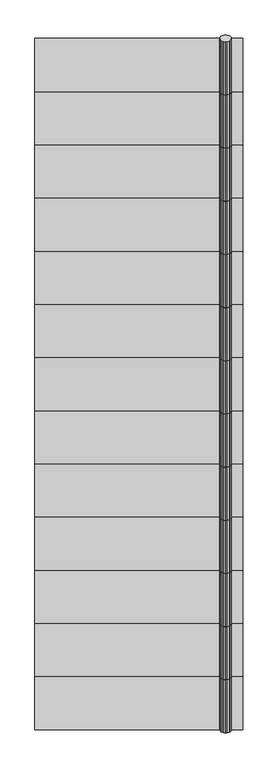
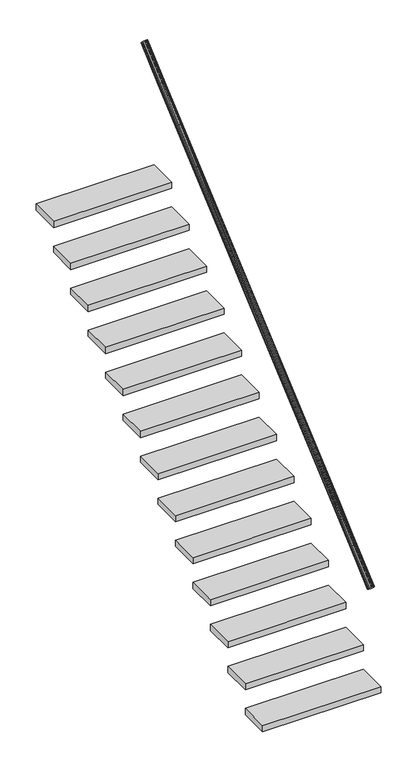
"""IFC4 building model written with IfcOpenShell, lengths in millimetres: stair geometry, 0_3d_modell."""

import ifcopenshell
import ifcopenshell.guid

model = None  # the IFC model being written
_history = None  # IfcOwnerHistory: only IFC2X3 demands one
_inside = {}  # id of a spatial element -> (the spatial element, [elements in it])
_under = {}  # id of a project, library or spatial element -> (it, [spatial elements below it])
_declared = {}  # id of a project -> (the project, [libraries it declares])
_typed = {}  # id of a type object -> (the type object, [elements of that type])
_made_of = {}  # id of a material, layer set ... -> (it, [elements and type objects made of it])


def new_model(schema):
    """Start an empty IFC model of exactly this schema.

    Asked for "IFC4X3", IfcOpenShell would pick the latest addendum, in which some entities
    have other attributes; the version numbers below select the first issue.
    IFC2X3 requires an IfcOwnerHistory on every rooted entity: one is made here for all.
    """
    global model, _history
    if schema == "IFC4X3":
        model = ifcopenshell.file(schema_version=(4, 3, 0, 0))
    else:
        model = ifcopenshell.file(schema=schema)
    _inside.clear()
    _under.clear()
    _declared.clear()
    _typed.clear()
    _made_of.clear()
    _history = None
    if model.schema == "IFC2X3":
        org = make("IfcOrganization", Name="unknown")
        user = make(
            "IfcPersonAndOrganization",
            ThePerson=make("IfcPerson", FamilyName="unknown"),
            TheOrganization=org,
        )
        app = make(
            "IfcApplication",
            ApplicationDeveloper=org,
            Version="unknown",
            ApplicationFullName="unknown",
            ApplicationIdentifier="unknown",
        )
        _history = make(
            "IfcOwnerHistory",
            OwningUser=user,
            OwningApplication=app,
            ChangeAction="ADDED",
            CreationDate=0,
        )
    return model


def make(cls, **values):
    """One entity of the class cls with the attributes given. An attribute that is None is left unset."""
    return model.create_entity(
        cls, **{name: value for name, value in values.items() if value is not None}
    )


def rooted(cls, **values):
    """An entity with a GlobalId (a new one), such as an element, a storey or a relation."""
    return make(cls, GlobalId=ifcopenshell.guid.new(), OwnerHistory=_history, **values)


def si_unit(unit_type, name, prefix=None):
    """IfcSIUnit, for example si_unit("LENGTHUNIT", "METRE", prefix="MILLI")."""
    return make("IfcSIUnit", UnitType=unit_type, Prefix=prefix, Name=name)


def assignment(units):
    """IfcUnitAssignment: the units of a project."""
    return None if units is None else make("IfcUnitAssignment", Units=units)


def point(xyz):
    """IfcCartesianPoint."""
    return None if xyz is None else make("IfcCartesianPoint", Coordinates=xyz)


def direction(xyz):
    """IfcDirection."""
    return None if xyz is None else make("IfcDirection", DirectionRatios=xyz)


def frame(location, z_axis=None, x_axis=None):
    """IfcAxis2Placement3D, a coordinate frame: its origin and axes. An axis left out is left unset."""
    return make(
        "IfcAxis2Placement3D",
        Location=point(location),
        Axis=direction(z_axis),
        RefDirection=direction(x_axis),
    )


def origin():
    """The frame at (0, 0, 0) with its axes left unset."""
    return frame((0.0, 0.0, 0.0))


def origin_with_axes():
    """The frame at (0, 0, 0) with the z axis (0, 0, 1) and the x axis (1, 0, 0) written out."""
    return frame((0.0, 0.0, 0.0), z_axis=(0.0, 0.0, 1.0), x_axis=(1.0, 0.0, 0.0))


def place(relative_to, where):
    """IfcLocalPlacement: puts the frame where relative to a parent placement (None: the world)."""
    return make(
        "IfcLocalPlacement", PlacementRelTo=relative_to, RelativePlacement=where
    )


def context(
    kind, dimensions, precision=None, world=None, true_north=None, identifier=None
):
    """IfcGeometricRepresentationContext, for example the 3D "Model" context."""
    return make(
        "IfcGeometricRepresentationContext",
        ContextIdentifier=identifier,
        ContextType=kind,
        CoordinateSpaceDimension=dimensions,
        Precision=precision,
        WorldCoordinateSystem=world,
        TrueNorth=true_north,
    )


def project(units=None, contexts=None):
    """IfcProject with its units and contexts."""
    return rooted(
        "IfcProject",
        Name="project",
        RepresentationContexts=contexts,
        UnitsInContext=assignment(units),
    )


def spatial(cls, under=None, at=None, **own):
    """A site, building, storey or space (cls), placed at a placement, below another one or the project."""
    s = rooted(cls, ObjectPlacement=at, **own)
    if under is not None:
        _under.setdefault(under.id(), (under, []))[1].append(s)
    return s


def polyline(points):
    """IfcPolyline through the points."""
    return make("IfcPolyline", Points=[point(p) for p in points])


def outline(outer, holes=None, kind="AREA"):
    """IfcArbitraryClosedProfileDef: a profile drawn as a closed curve; with holes, ...WithVoids."""
    if holes is None:
        return make("IfcArbitraryClosedProfileDef", ProfileType=kind, OuterCurve=outer)
    return make(
        "IfcArbitraryProfileDefWithVoids",
        ProfileType=kind,
        OuterCurve=outer,
        InnerCurves=holes,
    )


def extrude(swept, where, along, depth):
    """IfcExtrudedAreaSolid: the profile swept, set in the frame where, extruded along a direction by depth."""
    return make(
        "IfcExtrudedAreaSolid",
        SweptArea=swept,
        Position=where,
        ExtrudedDirection=direction(along),
        Depth=depth,
    )


def shape(context_of_items, identifier, shape_type, items):
    """IfcShapeRepresentation: the items that make up one representation, for example the "Body"."""
    return make(
        "IfcShapeRepresentation",
        ContextOfItems=context_of_items,
        RepresentationIdentifier=identifier,
        RepresentationType=shape_type,
        Items=items,
    )


def source(mapping_origin, context_of_items, identifier, shape_type, items):
    """IfcRepresentationMap: a shape defined once, which mapped items show again and again."""
    return make(
        "IfcRepresentationMap",
        MappingOrigin=mapping_origin,
        MappedRepresentation=shape(context_of_items, identifier, shape_type, items),
    )


def transform(
    local_origin,
    x_axis=None,
    y_axis=None,
    z_axis=None,
    scale=None,
    scale2=None,
    scale3=None,
    uniform=True,
):
    """IfcCartesianTransformationOperator3D, or its non-uniform kind. x_axis, y_axis, z_axis: its Axis1, 2, 3."""
    if uniform:
        return make(
            "IfcCartesianTransformationOperator3D",
            Axis1=direction(x_axis),
            Axis2=direction(y_axis),
            LocalOrigin=point(local_origin),
            Scale=scale,
            Axis3=direction(z_axis),
        )
    return make(
        "IfcCartesianTransformationOperator3DnonUniform",
        Axis1=direction(x_axis),
        Axis2=direction(y_axis),
        LocalOrigin=point(local_origin),
        Scale=scale,
        Axis3=direction(z_axis),
        Scale2=scale2,
        Scale3=scale3,
    )


def mapped(mapping_source, mapping_target):
    """IfcMappedItem: shows the shape of a source again, moved by a transform."""
    return make(
        "IfcMappedItem", MappingSource=mapping_source, MappingTarget=mapping_target
    )


def made_of(thing, what):
    """Note that an element or type object is made of a material, layer set ...; save() writes the relation."""
    if what is not None:
        _made_of.setdefault(what.id(), (what, []))[1].append(thing)
    return thing


def element(
    cls,
    number,
    at=None,
    inside=None,
    cuts=None,
    type_object=None,
    material=None,
    context=None,
    identifier="Body",
    shape_type=None,
    held_by="IfcProductDefinitionShape",
    body=None,
    shapes=None,
    **own,
):
    """One element of the class cls, such as IfcWall. Its Tag is "e" and its number.

    at: its placement. inside: the storey or other place that contains it. cuts: it is an
    opening in that element (IfcRelVoidsElement). A single representation is given by context,
    identifier, shape_type and body (its items); several are given by shapes. held_by: the class
    of the entity that holds the representations. save() writes the other relations.
    """
    e = rooted(cls, Tag="e%d" % number, ObjectPlacement=at, **own)
    if body is not None:
        shapes = [shape(context, identifier, shape_type, body)]
    if shapes is not None:
        e.Representation = make(held_by, Representations=shapes)
    if inside is not None:
        _inside.setdefault(inside.id(), (inside, []))[1].append(e)
    if cuts is not None:
        rooted(
            "IfcRelVoidsElement", RelatingBuildingElement=cuts, RelatedOpeningElement=e
        )
    if type_object is not None:
        _typed.setdefault(type_object.id(), (type_object, []))[1].append(e)
    return made_of(e, material)


def aggregate(whole, parts):
    """IfcRelAggregates: a whole, such as a stair, and the parts it consists of."""
    return rooted("IfcRelAggregates", RelatingObject=whole, RelatedObjects=parts)


def save(model, path):
    """Write the relations noted so far, then the file.

    IfcRelAggregates (storeys below a building ...), IfcRelContainedInSpatialStructure (elements
    in a storey), IfcRelDefinesByType, IfcRelAssociatesMaterial and IfcRelDeclares: one each for
    every whole, place, type object, material and project.
    """
    for whole, parts in _under.values():
        aggregate(whole, parts)
    for where, things in _inside.values():
        rooted(
            "IfcRelContainedInSpatialStructure",
            RelatedElements=things,
            RelatingStructure=where,
        )
    for kind, things in _typed.values():
        rooted("IfcRelDefinesByType", RelatedObjects=things, RelatingType=kind)
    for what, things in _made_of.values():
        rooted("IfcRelAssociatesMaterial", RelatedObjects=things, RelatingMaterial=what)
    for by, libraries in _declared.values():
        rooted("IfcRelDeclares", RelatingContext=by, RelatedDefinitions=libraries)
    model.write(path)


def stair_b80f565f(model_context):
    return source(origin(), model_context, "Body", "SweptSolid", [
        extrude(outline(polyline([(1.2235871, -7.0656631), (0.0, 0.0), (1.2235871, 7.065663), (4.7745751, 13.4396897), (10.3053687, 18.498146), (17.2745751, 21.7458748), (25.0, 22.8649659), (32.7254249, 21.7458748), (39.6946313, 18.498146), (45.2254249, 13.4396897), (48.7764129, 7.065663), (50.0, 0.0), (48.7764129, -7.0656631), (45.2254249, -13.4396898), (39.6946313, -18.498146), (32.7254249, -21.7458748), (25.0, -22.8649659), (17.2745751, -21.7458748), (10.3053687, -18.498146), (4.7745751, -13.4396898), (1.2235871, -7.0656631)])), frame((850.0, 2774.9421971, 3252.4163795), z_axis=(0.0, 0.7569287102857436, 0.6534974579485071), x_axis=(-1.0, 0.0, 0.0)), (0.0, 0.0, 1.0), 303.8595272),
        extrude(outline(polyline([(1.2235871, -7.0656631), (0.0, 0.0), (1.2235871, 7.065663), (4.7745751, 13.4396897), (10.3053687, 18.498146), (17.2745751, 21.7458748), (25.0, 22.8649659), (32.7254249, 21.7458748), (39.6946313, 18.498146), (45.2254249, 13.4396897), (48.7764129, 7.065663), (50.0, 0.0), (48.7764129, -7.0656631), (45.2254249, -13.4396898), (39.6946313, -18.498146), (32.7254249, -21.7458748), (25.0, -22.8649659), (17.2745751, -21.7458748), (10.3053687, -18.498146), (4.7745751, -13.4396898), (1.2235871, -7.0656631)])), frame((850.0, 1854.9421971, 2458.1306652), z_axis=(0.0, 0.7569287102857034, 0.6534974579485536), x_axis=(-1.0, 0.0, 0.0)), (0.0, 0.0, 1.0), 303.8595272),
        extrude(outline(polyline([(0.0, 2084.9421971), (0.0, 2314.9421971), (900.0, 2314.9421971), (900.0, 2084.9421971), (0.0, 2084.9421971)])), frame((0.0, 0.0, 1787.1428571), z_axis=(0.0, 0.0, 1.0), x_axis=(1.0, 0.0, 0.0)), (0.0, 0.0, 1.0), 50.0),
        extrude(outline(polyline([(0.0, 1394.9421971), (0.0, 1624.9421971), (900.0, 1624.9421971), (900.0, 1394.9421971), (0.0, 1394.9421971)])), frame((0.0, 0.0, 1191.4285714), z_axis=(0.0, 0.0, 1.0), x_axis=(1.0, 0.0, 0.0)), (0.0, 0.0, 1.0), 50.0),
        extrude(outline(polyline([(0.0, 14.9421971), (0.0, 244.9421971), (900.0, 244.9421971), (900.0, 14.9421971), (0.0, 14.9421971)])), origin_with_axes(), (0.0, 0.0, 1.0), 50.0),
        extrude(outline(polyline([(1.2235871, -7.0656631), (0.0, 0.0), (1.2235871, 7.0656631), (4.7745751, 13.4396898), (10.3053687, 18.4981461), (17.2745751, 21.7458748), (25.0, 22.8649659), (32.7254249, 21.7458748), (39.6946313, 18.4981461), (45.2254249, 13.4396898), (48.7764129, 7.0656631), (50.0, 0.0), (48.7764129, -7.0656631), (45.2254249, -13.4396897), (39.6946313, -18.498146), (32.7254249, -21.7458748), (25.0, -22.8649659), (17.2745751, -21.7458748), (10.3053687, -18.498146), (4.7745751, -13.4396897), (1.2235871, -7.0656631)])), frame((850.0, 474.9421971, 1266.7020937), z_axis=(0.0, 0.7569287102857089, 0.6534974579485475), x_axis=(-1.0, 0.0, 0.0)), (0.0, 0.0, 1.0), 303.8595272),
        extrude(outline(polyline([(0.0, 934.9421971), (0.0, 1164.9421971), (900.0, 1164.9421971), (900.0, 934.9421971), (0.0, 934.9421971)])), frame((0.0, 0.0, 794.2857143), z_axis=(0.0, 0.0, 1.0), x_axis=(1.0, 0.0, 0.0)), (0.0, 0.0, 1.0), 50.0),
        extrude(outline(polyline([(1.2235871, -7.0656631), (0.0, 0.0), (1.2235871, 7.065663), (4.7745751, 13.4396897), (10.3053687, 18.498146), (17.2745751, 21.7458748), (25.0, 22.8649659), (32.7254249, 21.7458748), (39.6946313, 18.498146), (45.2254249, 13.4396897), (48.7764129, 7.065663), (50.0, 0.0), (48.7764129, -7.0656631), (45.2254249, -13.4396897), (39.6946313, -18.498146), (32.7254249, -21.7458748), (25.0, -22.8649659), (17.2745751, -21.7458748), (10.3053687, -18.498146), (4.7745751, -13.4396897), (1.2235871, -7.0656631)])), frame((850.0, 14.9421971, 869.5592366), z_axis=(0.0, 0.7569287102857067, 0.6534974579485499), x_axis=(-1.0, 0.0, 0.0)), (0.0, 0.0, 1.0), 303.8595272),
        extrude(outline(polyline([(1.2235871, -7.0656631), (0.0, 0.0), (1.2235871, 7.065663), (4.7745751, 13.4396897), (10.3053687, 18.498146), (17.2745751, 21.7458748), (25.0, 22.8649659), (32.7254249, 21.7458748), (39.6946313, 18.498146), (45.2254249, 13.4396897), (48.7764129, 7.065663), (50.0, 0.0), (48.7764129, -7.0656631), (45.2254249, -13.4396897), (39.6946313, -18.498146), (32.7254249, -21.7458748), (25.0, -22.8649659), (17.2745751, -21.7458748), (10.3053687, -18.498146), (4.7745751, -13.4396897), (1.2235871, -7.0656631)])), frame((850.0, 1624.9421971, 2259.5592366), z_axis=(0.0, 0.7569287102856869, 0.653497457948573), x_axis=(-1.0, 0.0, 0.0)), (0.0, 0.0, 1.0), 303.8595272),
        extrude(outline(polyline([(1.2235871, -7.0656631), (0.0, 0.0), (1.2235871, 7.065663), (4.7745751, 13.4396897), (10.3053687, 18.498146), (17.2745751, 21.7458748), (25.0, 22.8649659), (32.7254249, 21.7458748), (39.6946313, 18.498146), (45.2254249, 13.4396897), (48.7764129, 7.065663), (50.0, 0.0), (48.7764129, -7.0656631), (45.2254249, -13.4396898), (39.6946313, -18.498146), (32.7254249, -21.7458748), (25.0, -22.8649659), (17.2745751, -21.7458748), (10.3053687, -18.498146), (4.7745751, -13.4396898), (1.2235871, -7.0656631)])), frame((850.0, 1164.9421971, 1862.4163795), z_axis=(0.0, 0.7569287102857021, 0.6534974579485554), x_axis=(-1.0, 0.0, 0.0)), (0.0, 0.0, 1.0), 303.8595272),
        extrude(outline(polyline([(1.2235871, -7.0656631), (0.0, 0.0), (1.2235871, 7.065663), (4.7745751, 13.4396897), (10.3053687, 18.498146), (17.2745751, 21.7458748), (25.0, 22.8649659), (32.7254249, 21.7458748), (39.6946313, 18.498146), (45.2254249, 13.4396897), (48.7764129, 7.065663), (50.0, 0.0), (48.7764129, -7.0656631), (45.2254249, -13.4396898), (39.6946313, -18.498146), (32.7254249, -21.7458748), (25.0, -22.8649659), (17.2745751, -21.7458748), (10.3053687, -18.498146), (4.7745751, -13.4396898), (1.2235871, -7.0656631)])), frame((850.0, 934.9421971, 1663.8449509), z_axis=(0.0, 0.7569287102857098, 0.6534974579485463), x_axis=(-1.0, 0.0, 0.0)), (0.0, 0.0, 1.0), 303.8595272),
        extrude(outline(polyline([(0.0, 1164.9421971), (0.0, 1394.9421971), (900.0, 1394.9421971), (900.0, 1164.9421971), (0.0, 1164.9421971)])), frame((0.0, 0.0, 992.8571429), z_axis=(0.0, 0.0, 1.0), x_axis=(1.0, 0.0, 0.0)), (0.0, 0.0, 1.0), 50.0),
        extrude(outline(polyline([(1.2235871, -7.0656631), (0.0, 0.0), (1.2235871, 7.065663), (4.7745751, 13.4396897), (10.3053687, 18.498146), (17.2745751, 21.7458748), (25.0, 22.8649659), (32.7254249, 21.7458748), (39.6946313, 18.498146), (45.2254249, 13.4396897), (48.7764129, 7.065663), (50.0, 0.0), (48.7764129, -7.0656631), (45.2254249, -13.4396898), (39.6946313, -18.498146), (32.7254249, -21.7458748), (25.0, -22.8649659), (17.2745751, -21.7458748), (10.3053687, -18.498146), (4.7745751, -13.4396898), (1.2235871, -7.0656631)])), frame((850.0, 244.9421971, 1068.1306652), z_axis=(0.0, 0.7569287102856895, 0.6534974579485698), x_axis=(-1.0, 0.0, 0.0)), (0.0, 0.0, 1.0), 303.8595272),
        extrude(outline(polyline([(0.0, 244.9421971), (0.0, 474.9421971), (900.0, 474.9421971), (900.0, 244.9421971), (0.0, 244.9421971)])), frame((0.0, 0.0, 198.5714286), z_axis=(0.0, 0.0, 1.0), x_axis=(1.0, 0.0, 0.0)), (0.0, 0.0, 1.0), 50.0),
        extrude(outline(polyline([(1.2235871, -7.0656631), (0.0, 0.0), (1.2235871, 7.065663), (4.7745751, 13.4396897), (10.3053687, 18.498146), (17.2745751, 21.7458748), (25.0, 22.8649659), (32.7254249, 21.7458748), (39.6946313, 18.498146), (45.2254249, 13.4396897), (48.7764129, 7.065663), (50.0, 0.0), (48.7764129, -7.0656631), (45.2254249, -13.4396898), (39.6946313, -18.498146), (32.7254249, -21.7458748), (25.0, -22.8649659), (17.2745751, -21.7458748), (10.3053687, -18.498146), (4.7745751, -13.4396898), (1.2235871, -7.0656631)])), frame((850.0, 2544.9421971, 3053.8449509), z_axis=(0.0, 0.7569287102857051, 0.6534974579485517), x_axis=(-1.0, 0.0, 0.0)), (0.0, 0.0, 1.0), 303.8595272),
        extrude(outline(polyline([(1.2235871, -7.0656631), (0.0, 0.0), (1.2235871, 7.0656631), (4.7745751, 13.4396898), (10.3053687, 18.4981461), (17.2745751, 21.7458748), (25.0, 22.8649659), (32.7254249, 21.7458748), (39.6946313, 18.4981461), (45.2254249, 13.4396898), (48.7764129, 7.0656631), (50.0, 0.0), (48.7764129, -7.0656631), (45.2254249, -13.4396897), (39.6946313, -18.498146), (32.7254249, -21.7458748), (25.0, -22.8649659), (17.2745751, -21.7458748), (10.3053687, -18.498146), (4.7745751, -13.4396897), (1.2235871, -7.0656631)])), frame((850.0, 2084.9421971, 2656.7020937), z_axis=(0.0, 0.7569287102856951, 0.6534974579485633), x_axis=(-1.0, 0.0, 0.0)), (0.0, 0.0, 1.0), 303.8595272),
        extrude(outline(polyline([(0.0, 1624.9421971), (0.0, 1854.9421971), (900.0, 1854.9421971), (900.0, 1624.9421971), (0.0, 1624.9421971)])), frame((0.0, 0.0, 1390.0), z_axis=(0.0, 0.0, 1.0), x_axis=(1.0, 0.0, 0.0)), (0.0, 0.0, 1.0), 50.0),
        extrude(outline(polyline([(0.0, 704.9421971), (0.0, 934.9421971), (900.0, 934.9421971), (900.0, 704.9421971), (0.0, 704.9421971)])), frame((0.0, 0.0, 595.7142857), z_axis=(0.0, 0.0, 1.0), x_axis=(1.0, 0.0, 0.0)), (0.0, 0.0, 1.0), 50.0),
        extrude(outline(polyline([(0.0, 474.9421971), (0.0, 704.9421971), (900.0, 704.9421971), (900.0, 474.9421971), (0.0, 474.9421971)])), frame((0.0, 0.0, 397.1428571), z_axis=(0.0, 0.0, 1.0), x_axis=(1.0, 0.0, 0.0)), (0.0, 0.0, 1.0), 50.0),
        extrude(outline(polyline([(0.0, 2314.9421971), (0.0, 2544.9421971), (900.0, 2544.9421971), (900.0, 2314.9421971), (0.0, 2314.9421971)])), frame((0.0, 0.0, 1985.7142857), z_axis=(0.0, 0.0, 1.0), x_axis=(1.0, 0.0, 0.0)), (0.0, 0.0, 1.0), 50.0),
        extrude(outline(polyline([(1.2235871, -7.0656631), (0.0, 0.0), (1.2235871, 7.065663), (4.7745751, 13.4396898), (10.3053687, 18.498146), (17.2745751, 21.7458748), (25.0, 22.8649659), (32.7254249, 21.7458748), (39.6946313, 18.498146), (45.2254249, 13.4396898), (48.7764129, 7.065663), (50.0, 0.0), (48.7764129, -7.0656631), (45.2254249, -13.4396897), (39.6946313, -18.498146), (32.7254249, -21.7458748), (25.0, -22.8649659), (17.2745751, -21.7458748), (10.3053687, -18.498146), (4.7745751, -13.4396897), (1.2235871, -7.0656631)])), frame((850.0, 704.9421971, 1465.2735223), z_axis=(0.0, 0.7569287102857089, 0.6534974579485475), x_axis=(-1.0, 0.0, 0.0)), (0.0, 0.0, 1.0), 303.8595272),
        extrude(outline(polyline([(0.0, 2774.9421971), (0.0, 3004.9421971), (900.0, 3004.9421971), (900.0, 2774.9421971), (0.0, 2774.9421971)])), frame((0.0, 0.0, 2382.8571429), z_axis=(0.0, 0.0, 1.0), x_axis=(1.0, 0.0, 0.0)), (0.0, 0.0, 1.0), 50.0),
        extrude(outline(polyline([(0.0, 1854.9421971), (0.0, 2084.9421971), (900.0, 2084.9421971), (900.0, 1854.9421971), (0.0, 1854.9421971)])), frame((0.0, 0.0, 1588.5714286), z_axis=(0.0, 0.0, 1.0), x_axis=(1.0, 0.0, 0.0)), (0.0, 0.0, 1.0), 50.0),
        extrude(outline(polyline([(0.0, 2544.9421971), (0.0, 2774.9421971), (900.0, 2774.9421971), (900.0, 2544.9421971), (0.0, 2544.9421971)])), frame((0.0, 0.0, 2184.2857143), z_axis=(0.0, 0.0, 1.0), x_axis=(1.0, 0.0, 0.0)), (0.0, 0.0, 1.0), 50.0),
        extrude(outline(polyline([(1.2235871, -7.0656631), (0.0, 0.0), (1.2235871, 7.065663), (4.7745751, 13.4396898), (10.3053687, 18.498146), (17.2745751, 21.7458748), (25.0, 22.8649659), (32.7254249, 21.7458748), (39.6946313, 18.498146), (45.2254249, 13.4396898), (48.7764129, 7.065663), (50.0, 0.0), (48.7764129, -7.0656631), (45.2254249, -13.4396897), (39.6946313, -18.498146), (32.7254249, -21.7458748), (25.0, -22.8649659), (17.2745751, -21.7458748), (10.3053687, -18.498146), (4.7745751, -13.4396897), (1.2235871, -7.0656631)])), frame((850.0, 2314.9421971, 2855.2735223), z_axis=(0.0, 0.7569287102856991, 0.6534974579485587), x_axis=(-1.0, 0.0, 0.0)), (0.0, 0.0, 1.0), 303.8595272),
        extrude(outline(polyline([(1.2235871, -7.0656631), (0.0, 0.0), (1.2235871, 7.0656631), (4.7745751, 13.4396898), (10.3053687, 18.498146), (17.2745751, 21.7458748), (25.0, 22.8649659), (32.7254249, 21.7458748), (39.6946313, 18.498146), (45.2254249, 13.4396898), (48.7764129, 7.0656631), (50.0, 0.0), (48.7764129, -7.0656631), (45.2254249, -13.4396897), (39.6946313, -18.498146), (32.7254249, -21.7458748), (25.0, -22.8649659), (17.2745751, -21.7458748), (10.3053687, -18.498146), (4.7745751, -13.4396897), (1.2235871, -7.0656631)])), frame((850.0, 1394.9421971, 2060.987808), z_axis=(0.0, 0.7569287102857012, 0.6534974579485563), x_axis=(-1.0, 0.0, 0.0)), (0.0, 0.0, 1.0), 303.8595272),
    ])


if __name__ == "__main__":
    model = new_model("IFC4")
    model_context = context("Model", 3, world=origin())
    ifc_project = project(units=[si_unit("LENGTHUNIT", "METRE", prefix="MILLI")], contexts=[model_context])
    site = spatial("IfcSite", under=ifc_project)
    building = spatial("IfcBuilding", under=site)
    placement = place(None, origin())
    stair_shape = stair_b80f565f(model_context)
    element("IfcStair", 1, ObjectType="0_3d_modell", at=placement, inside=building, context=model_context, shape_type="MappedRepresentation", body=[
        mapped(stair_shape, transform((0.0, 0.0, 0.0), x_axis=(1.0, 0.0, 0.0), y_axis=(0.0, 1.0, 0.0), z_axis=(0.0, 0.0, 1.0))),
    ])
    save(model, "model.ifc")

# Revit data of these elements
# Element 1 (IfcStair, "0_3d_modell")
#   Materials on its faces: "*1", "weiss"
# Materials
#   "*1": class "Unassigned", colour RGB 175 175 175, transparency 0
#   "weiss": class "Unassigned", colour RGB 255 255 255, transparency 0
